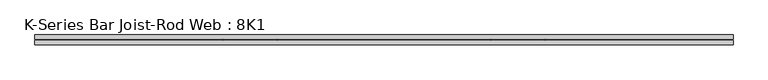
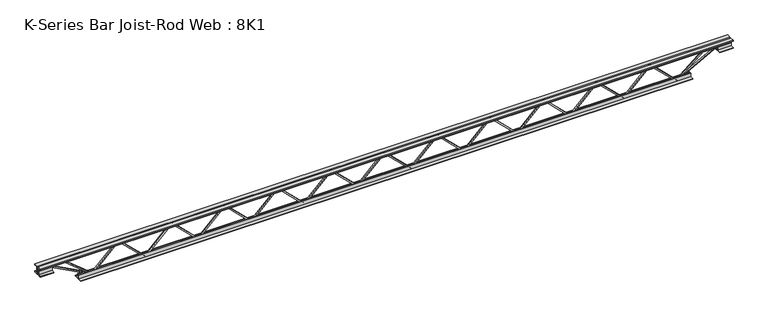
"""IFC4 building model written with IfcOpenShell, lengths in millimetres: beam geometry, K-Series Bar Joist-Rod Web : 8K1."""

from ifc_helpers import new_model, si_unit, frame, origin, place, context, project, spatial, polyline, outline, extrude, source, transform, mapped, element, save


def k_series_bar_joist_rod_web_8k1_3393dd89(model_context):
    return source(origin(), model_context, "Body", "SweptSolid", [
        extrude(outline(polyline([(-90.4875, 1404.3922228), (-100.0125, 1404.3922228), (-100.0125, 1409.5125828), (90.4875, 1603.7900432), (90.4875, 1606.2493231), (-100.0125, 1800.5267835), (-100.0125, 1805.6471436), (-90.4875, 1805.6471436), (-90.4875, 1804.4175036), (100.0125, 1610.1400432), (100.0125, 1599.8993231), (-90.4875, 1405.6218627), (-90.4875, 1404.3922228)])), frame((0.0, -4.7625, 0.0), z_axis=(0.0, 1.0, 0.0), x_axis=(0.0, 0.0, 1.0)), (0.0, 0.0, 1.0), 9.525),
        extrude(outline(polyline([(-90.4875, 1003.137302), (-100.0125, 1003.137302), (-100.0125, 1008.257662), (90.4875, 1202.5351224), (90.4875, 1204.9944023), (-100.0125, 1399.2718627), (-100.0125, 1404.3922228), (-90.4875, 1404.3922228), (-90.4875, 1403.1625828), (100.0125, 1208.8851224), (100.0125, 1198.6444023), (-90.4875, 1004.3669419), (-90.4875, 1003.137302)])), frame((0.0, -4.7625, 0.0), z_axis=(0.0, 1.0, 0.0), x_axis=(0.0, 0.0, 1.0)), (0.0, 0.0, 1.0), 9.525),
        extrude(outline(polyline([(-90.4875, 601.8823812), (-100.0125, 601.8823812), (-100.0125, 607.0027412), (90.4875, 801.2802016), (90.4875, 803.7394815), (-100.0125, 998.0169419), (-100.0125, 1003.137302), (-90.4875, 1003.137302), (-90.4875, 1001.907662), (100.0125, 807.6302016), (100.0125, 797.3894815), (-90.4875, 603.1120211), (-90.4875, 601.8823812)])), frame((0.0, -4.7625, 0.0), z_axis=(0.0, 1.0, 0.0), x_axis=(0.0, 0.0, 1.0)), (0.0, 0.0, 1.0), 9.525),
        extrude(outline(polyline([(-90.4875, 200.6274604), (-100.0125, 200.6274604), (-100.0125, 205.7478205), (90.4875, 400.0252809), (90.4875, 402.4845607), (-100.0125, 596.7620211), (-100.0125, 601.8823812), (-90.4875, 601.8823812), (-90.4875, 600.6527412), (100.0125, 406.3752809), (100.0125, 396.1345607), (-90.4875, 201.8571003), (-90.4875, 200.6274604)])), frame((0.0, -4.7625, 0.0), z_axis=(0.0, 1.0, 0.0), x_axis=(0.0, 0.0, 1.0)), (0.0, 0.0, 1.0), 9.525),
        extrude(outline(polyline([(-90.4875, -200.6274604), (-100.0125, -200.6274604), (-100.0125, -195.5071003), (90.4875, -1.2296399), (90.4875, 1.2296399), (-100.0125, 195.5071003), (-100.0125, 200.6274604), (-90.4875, 200.6274604), (-90.4875, 199.3978205), (100.0125, 5.1203601), (100.0125, -5.1203601), (-90.4875, -199.3978205), (-90.4875, -200.6274604)])), frame((0.0, -4.7625, 0.0), z_axis=(0.0, 1.0, 0.0), x_axis=(0.0, 0.0, 1.0)), (0.0, 0.0, 1.0), 9.525),
        extrude(outline(polyline([(-90.4875, -601.8823812), (-100.0125, -601.8823812), (-100.0125, -596.7620211), (90.4875, -402.4845607), (90.4875, -400.0252809), (-100.0125, -205.7478205), (-100.0125, -200.6274604), (-90.4875, -200.6274604), (-90.4875, -201.8571003), (100.0125, -396.1345607), (100.0125, -406.3752809), (-90.4875, -600.6527412), (-90.4875, -601.8823812)])), frame((0.0, -4.7625, 0.0), z_axis=(0.0, 1.0, 0.0), x_axis=(0.0, 0.0, 1.0)), (0.0, 0.0, 1.0), 9.525),
        extrude(outline(polyline([(-90.4875, -1003.137302), (-100.0125, -1003.137302), (-100.0125, -998.0169419), (90.4875, -803.7394815), (90.4875, -801.2802016), (-100.0125, -607.0027412), (-100.0125, -601.8823812), (-90.4875, -601.8823812), (-90.4875, -603.1120211), (100.0125, -797.3894815), (100.0125, -807.6302016), (-90.4875, -1001.907662), (-90.4875, -1003.137302)])), frame((0.0, -4.7625, 0.0), z_axis=(0.0, 1.0, 0.0), x_axis=(0.0, 0.0, 1.0)), (0.0, 0.0, 1.0), 9.525),
        extrude(outline(polyline([(-90.4875, -1404.3922228), (-100.0125, -1404.3922228), (-100.0125, -1399.2718627), (90.4875, -1204.9944023), (90.4875, -1202.5351224), (-100.0125, -1008.257662), (-100.0125, -1003.137302), (-90.4875, -1003.137302), (-90.4875, -1004.3669419), (100.0125, -1198.6444023), (100.0125, -1208.8851224), (-90.4875, -1403.1625828), (-90.4875, -1404.3922228)])), frame((0.0, -4.7625, 0.0), z_axis=(0.0, 1.0, 0.0), x_axis=(0.0, 0.0, 1.0)), (0.0, 0.0, 1.0), 9.525),
        extrude(outline(polyline([(-90.4875, -1805.6471436), (-100.0125, -1805.6471436), (-100.0125, -1800.5267835), (90.4875, -1606.2493231), (90.4875, -1603.7900432), (-100.0125, -1409.5125828), (-100.0125, -1404.3922228), (-90.4875, -1404.3922228), (-90.4875, -1405.6218627), (100.0125, -1599.8993231), (100.0125, -1610.1400432), (-90.4875, -1804.4175036), (-90.4875, -1805.6471436)])), frame((0.0, -4.7625, 0.0), z_axis=(0.0, 1.0, 0.0), x_axis=(0.0, 0.0, 1.0)), (0.0, 0.0, 1.0), 9.525),
        extrude(outline(polyline([(-90.4875, 1805.6471436), (-100.0125, 1805.6471436), (-100.0125, 1810.7675036), (90.4875, 2005.044964), (90.4875, 2007.5042439), (-100.0125, 2201.7817043), (-100.0125, 2206.9020644), (-90.4875, 2206.9020644), (-90.4875, 2205.6724244), (100.0125, 2011.394964), (100.0125, 2001.1542439), (-90.4875, 1806.8767835), (-90.4875, 1805.6471436)])), frame((0.0, -4.7625, 0.0), z_axis=(0.0, 1.0, 0.0), x_axis=(0.0, 0.0, 1.0)), (0.0, 0.0, 1.0), 9.525),
        extrude(outline(polyline([(-90.4875, -2206.9020644), (-100.0125, -2206.9020644), (-100.0125, -2201.7817043), (90.4875, -2007.5042439), (90.4875, -2005.044964), (-100.0125, -1810.7675036), (-100.0125, -1805.6471436), (-90.4875, -1805.6471436), (-90.4875, -1806.8767835), (100.0125, -2001.1542439), (100.0125, -2011.394964), (-90.4875, -2205.6724244), (-90.4875, -2206.9020644)])), frame((0.0, -4.7625, 0.0), z_axis=(0.0, 1.0, 0.0), x_axis=(0.0, 0.0, 1.0)), (0.0, 0.0, 1.0), 9.525),
        extrude(outline(polyline([(4.7625, 101.6), (36.5125, 101.6), (36.5125, 95.25), (11.1125, 95.25), (11.1125, 69.85), (4.7625, 69.85), (4.7625, 101.6)])), frame((-2613.3020644, 0.0, 0.0), z_axis=(1.0, 0.0, 0.0), x_axis=(0.0, 1.0, 0.0)), (0.0, 0.0, 1.0), 5226.6041288),
        extrude(outline(polyline([(-4.7625, 101.6), (-4.7625, 69.85), (-11.1125, 69.85), (-11.1125, 95.25), (-36.5125, 95.25), (-36.5125, 101.6), (-4.7625, 101.6)])), frame((-2613.3020644, 0.0, 0.0), z_axis=(1.0, 0.0, 0.0), x_axis=(0.0, 1.0, 0.0)), (0.0, 0.0, 1.0), 5226.6041288),
        extrude(outline(polyline([(-4.7625, 38.1), (-36.5125, 38.1), (-36.5125, 44.45), (-11.1125, 44.45), (-11.1125, 69.85), (-4.7625, 69.85), (-4.7625, 38.1)])), frame((-2613.3020644, 0.0, 0.0), z_axis=(1.0, 0.0, 0.0), x_axis=(0.0, 1.0, 0.0)), (0.0, 0.0, 1.0), 101.6),
        extrude(outline(polyline([(36.5125, 38.1), (4.7625, 38.1), (4.7625, 69.85), (11.1125, 69.85), (11.1125, 44.45), (36.5125, 44.45), (36.5125, 38.1)])), frame((-2613.3020644, 0.0, 0.0), z_axis=(1.0, 0.0, 0.0), x_axis=(0.0, 1.0, 0.0)), (0.0, 0.0, 1.0), 101.6),
        extrude(outline(polyline([(4.7625, 38.1), (4.7625, 69.85), (11.1125, 69.85), (11.1125, 44.45), (36.5125, 44.45), (36.5125, 38.1), (4.7625, 38.1)])), frame((2511.7020644, 0.0, 0.0), z_axis=(1.0, 0.0, 0.0), x_axis=(0.0, 1.0, 0.0)), (0.0, 0.0, 1.0), 101.6),
        extrude(outline(polyline([(-4.7625, 38.1), (-36.5125, 38.1), (-36.5125, 44.45), (-11.1125, 44.45), (-11.1125, 69.85), (-4.7625, 69.85), (-4.7625, 38.1)])), frame((2511.7020644, 0.0, 0.0), z_axis=(1.0, 0.0, 0.0), x_axis=(0.0, 1.0, 0.0)), (0.0, 0.0, 1.0), 101.6),
        extrude(outline(polyline([(4.7625, -101.6), (4.7625, -69.85), (11.1125, -69.85), (11.1125, -95.25), (36.5125, -95.25), (36.5125, -101.6), (4.7625, -101.6)])), frame((-2308.5020644, 0.0, 0.0), z_axis=(1.0, 0.0, 0.0), x_axis=(0.0, 1.0, 0.0)), (0.0, 0.0, 1.0), 4617.0041288),
        extrude(outline(polyline([(-4.7625, -101.6), (-36.5125, -101.6), (-36.5125, -95.25), (-11.1125, -95.25), (-11.1125, -69.85), (-4.7625, -69.85), (-4.7625, -101.6)])), frame((-2308.5020644, 0.0, 0.0), z_axis=(1.0, 0.0, 0.0), x_axis=(0.0, 1.0, 0.0)), (0.0, 0.0, 1.0), 4617.0041288),
        extrude(outline(polyline([(0.0, -9.525), (0.0, 0.0), (346.6425392, 0.0), (346.6425392, -9.525), (0.0, -9.525)])), frame((-2513.9703629, 4.7625, 65.662372), z_axis=(0.47628314854008025, 0.0, 0.8792919665371383), x_axis=(0.8792919665371383, 0.0, -0.47628314854008025)), (0.0, 0.0, 1.0), 9.525),
        extrude(outline(polyline([(0.0, -9.525), (0.0, 0.0), (259.8256875, 0.0), (259.8256875, -9.525), (0.0, -9.525)])), frame((-2410.5557412, 4.7625, 66.1725796), z_axis=(0.635426010457683, 0.0, 0.7721617610538822), x_axis=(0.7721617610538822, 0.0, -0.635426010457683)), (0.0, 0.0, 1.0), 9.525),
        extrude(outline(polyline([(0.0, -9.525), (0.0, 0.0), (346.6425392, 0.0), (346.6425392, -9.525), (0.0, -9.525)])), frame((2513.9703629, -4.7625, 65.662372), z_axis=(-0.4762831485400441, 0.0, 0.8792919665371579), x_axis=(-0.8792919665371579, 0.0, -0.4762831485400441)), (0.0, 0.0, 1.0), 9.525),
        extrude(outline(polyline([(0.0, -9.525), (0.0, 0.0), (259.8256875, 0.0), (259.8256875, -9.525), (0.0, -9.525)])), frame((2410.5557412, -4.7625, 66.1725796), z_axis=(-0.6354260104576576, 0.0, 0.772161761053903), x_axis=(-0.772161761053903, 0.0, -0.6354260104576576)), (0.0, 0.0, 1.0), 9.525),
    ])


if __name__ == "__main__":
    model = new_model("IFC4")
    model_context = context("Model", 3, world=origin())
    ifc_project = project(units=[si_unit("LENGTHUNIT", "METRE", prefix="MILLI")], contexts=[model_context])
    site = spatial("IfcSite", under=ifc_project)
    building = spatial("IfcBuilding", under=site)
    placement = place(None, origin())
    k_series_bar_joist_rod_web_8k1_shape = k_series_bar_joist_rod_web_8k1_3393dd89(model_context)
    element("IfcBeam", 1, ObjectType="K-Series Bar Joist-Rod Web : 8K1", at=placement, inside=building, context=model_context, shape_type="MappedRepresentation", body=[
        mapped(k_series_bar_joist_rod_web_8k1_shape, transform((0.0, 0.0, 0.0), x_axis=(1.0, 0.0, 0.0), y_axis=(0.0, 1.0, 0.0), z_axis=(0.0, 0.0, 1.0))),
    ])
    save(model, "model.ifc")

# Revit data of these elements
# Type "K-Series Bar Joist-Rod Web : 8K1"
#   Assembly Code = "B1010350"
#   Wt = 5.1
#   Web Thickness = 0' - 0 3/8"
#   Start Offset [instance default] = 0' - 0"
#   Start Extension [instance default] = 0' - 0"
#   Seat Length = 0' - 4"
#   Seat Depth = 0' - 2 1/2"
#   PanelArrayLength [instance default] = 21' - 4"
#   Panel [instance default] = 1' - 4"
#   End Offset [instance default] = 0' - 0"
#   End Extension [instance default] = 0' - 0"
#   End Panel = 1' - 4"
#   Cord Leg = 0' - 1 1/4"
#   Chord Thickness = 0' - 0 1/4"
#   Length [instance default] = 24' - 0"
#   Depth = 0' - 8"
#   PanelArrayNum [instance default] = 16
#   Rendering Material = none
# Element 1 (IfcBeam, "K-Series Bar Joist-Rod Web : 8K1")
#   PanelArrayLength = 14' - 5.77182"
#   Panel = 1' - 3.79744"
#   PanelArrayNum = 11
